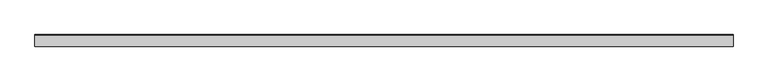
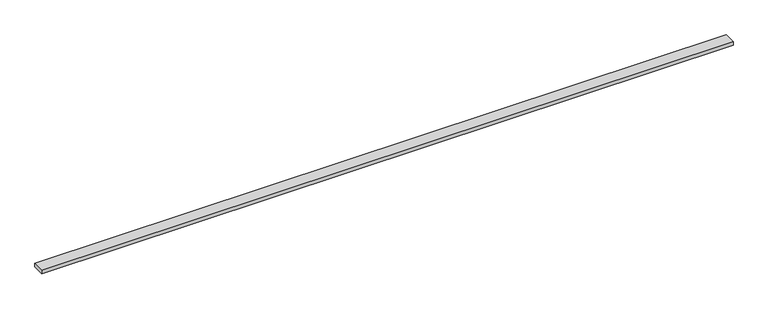
"""IFC4 building model written with IfcOpenShell, lengths in millimetres: proxy geometry, Inner panel:Inner panel:1:Inner panel:1 : Inner panel:Inner panel:300324:2:Inner panel:1:Inner panel:1 : Inner panel:Inner panel:300324:2 : Inner panel:Inner panel:1:Inner panel:1 : Inner panel:Inner panel:300324:300043:3 : Inner panel:Inner panel:1:Inner panel:1 : Inner panel:Inner panel:300324:2:Inner panel:1:Inner panel:1 : Inner panel:Inner panel:300324:2 : Inner panel:Inner panel:1:Inner panel:1 : Inner panel:Inner panel:300324:300043:308120."""

from ifc_helpers import new_model, si_unit, frame, origin, place, context, project, spatial, polyline, outline, extrude, source, transform, mapped, element, save


def generic_models_ff159b71(model_context):
    return source(origin(), model_context, "Body", "SweptSolid", [
        extrude(outline(polyline([(0.0, -80.594733), (0.0, 0.0), (4876.8, 0.0), (4876.8, -80.594733), (0.0, -80.594733)])), frame((596182.8367239, -575614.9038959, 4065.5507911), z_axis=(0.0, -0.04163054471214556, 0.9991330730923534), x_axis=(-1.0, 0.0, 0.0)), (0.0, 0.0, 1.0), 25.4),
    ])


if __name__ == "__main__":
    model = new_model("IFC4")
    model_context = context("Model", 3, world=origin())
    ifc_project = project(units=[si_unit("LENGTHUNIT", "METRE", prefix="MILLI")], contexts=[model_context])
    site = spatial("IfcSite", under=ifc_project)
    building = spatial("IfcBuilding", under=site)
    placement = place(None, origin())
    generic_models_shape = generic_models_ff159b71(model_context)
    element("IfcBuildingElementProxy", 1, Name="Inner panel:Inner panel:1:Inner panel:1 : Inner panel:Inner panel:300324:2:Inner panel:1:Inner panel:1 : Inner panel:Inner panel:300324:2 : Inner panel:Inner panel:1:Inner panel:1 : Inner panel:Inner panel:300324:300043:3 : Inner panel:Inner panel:1:Inner panel:1 : Inner panel:Inner panel:300324:2:Inner panel:1:Inner panel:1 : Inner panel:Inner panel:300324:2 : Inner panel:Inner panel:1:Inner panel:1 : Inner panel:Inner panel:300324:300043:308120", ObjectType="Inner panel:Inner panel:1:Inner panel:1 : Inner panel:Inner panel:300324:2:Inner panel:1:Inner panel:1 : Inner panel:Inner panel:300324:2 : Inner panel:Inner panel:1:Inner panel:1 : Inner panel:Inner panel:300324:300043:3 : Inner panel:Inner panel:1:Inner panel:1 : Inner panel:Inner panel:300324:2:Inner panel:1:Inner panel:1 : Inner panel:Inner panel:300324:2 : Inner panel:Inner panel:1:Inner panel:1 : Inner panel:Inner panel:300324:300043:308120", at=placement, inside=building, context=model_context, shape_type="MappedRepresentation", body=[
        mapped(generic_models_shape, transform((0.0, 0.0, 0.0), x_axis=(1.0, 0.0, 0.0), y_axis=(0.0, 1.0, 0.0), z_axis=(0.0, 0.0, 1.0))),
    ])
    save(model, "model.ifc")

# Revit data of these elements
# Type "Inner panel:Inner panel:1:Inner panel:1 : Inner panel:Inner panel:300324:2:Inner panel:1:Inner panel:1 : Inner panel:Inner panel:300324:2 : Inner panel:Inner panel:1:Inner panel:1 : Inner panel:Inner panel:300324:300043:3 : Inner panel:Inner panel:1:Inner panel:1 : Inner panel:Inner panel:300324:2:Inner panel:1:Inner panel:1 : Inner panel:Inner panel:300324:2 : Inner panel:Inner panel:1:Inner panel:1 : Inner panel:Inner panel:300324:300043:308120"
#   NameOverride = "Inner panel:Inner panel:1:Inner panel:1 : Inner panel:Inner panel:300324:2:Inner panel:1:Inner panel:1 : Inner panel:Inner panel:300324:2 : Inner panel:Inner panel:1:Inner panel:1 : Inner panel:Inner panel:300324:300043:308120"
#   ObjectTypeOverride = "Inner panel:1:Inner panel:1 : Inner panel:Inner panel:300324:2 : Inner panel:Inner panel:1:Inner panel:1 : Inner panel:Inner panel:300324:300043"
#   Reference = "Inner panel"
#   Tag = "308120"
# Element 1 (IfcBuildingElementProxy, "Inner panel:Inner panel:1:Inner panel:1 : Inner panel:Inner panel:300324:2:Inner panel:1:Inner panel:1 : Inner panel:Inner panel:300324:2 : Inner panel:Inner panel:1:Inner panel:1 : Inner panel:Inner panel:300324:300043:3 : Inner panel:Inner panel:1:Inner panel:1 : Inner panel:Inner panel:300324:2:Inner panel:1:Inner panel:1 : Inner panel:Inner panel:300324:2 : Inner panel:Inner panel:1:Inner panel:1 : Inner panel:Inner panel:300324:300043:308120")
#   Materials on its faces: "1\" THERMAL SPACER @ PURLIN"
# Materials
#   "1\" THERMAL SPACER @ PURLIN": class "Unassigned", colour RGB 205 188 106, transparency 0, Cost = 0
